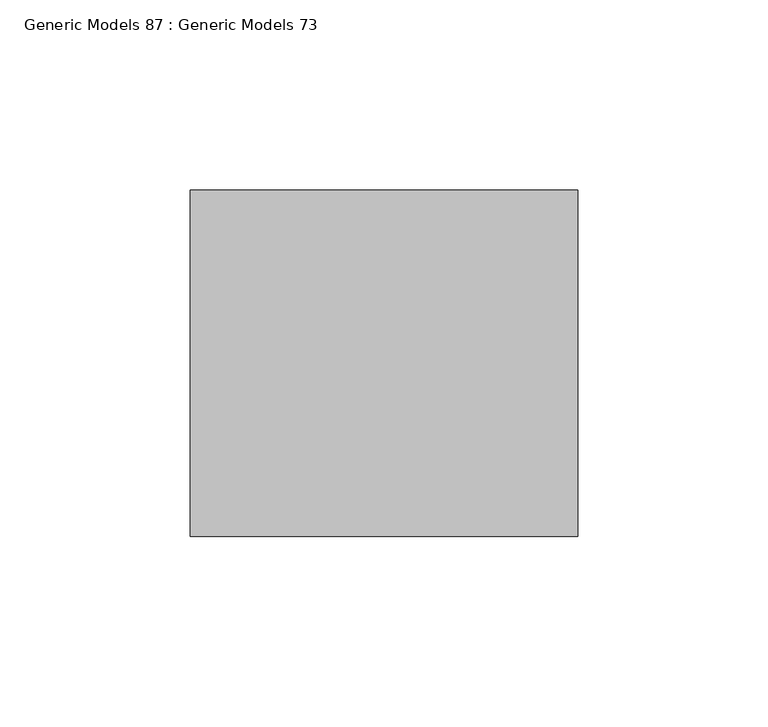
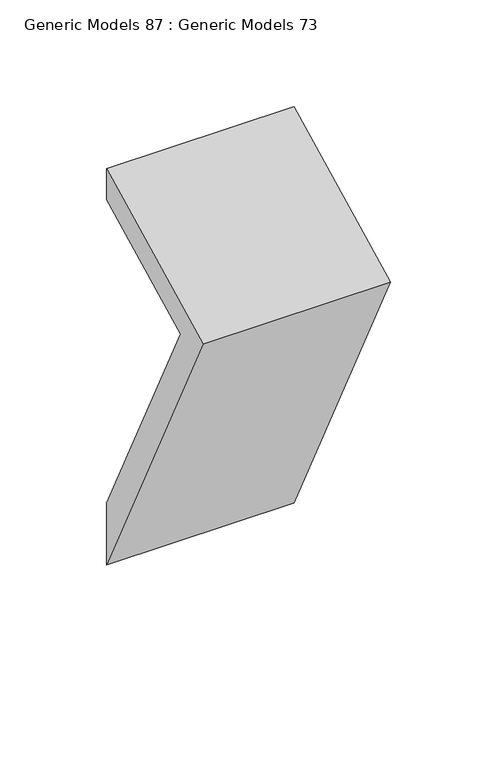
"""IFC4 building model written with IfcOpenShell, lengths in millimetres: proxy geometry, Generic Models 87 : Generic Models 73."""

from ifc_helpers import new_model, si_unit, frame, origin, place, context, project, spatial, polyline, outline, extrude, source, transform, mapped, element, save


def generic_models_87_generic_models_73_a56742e6(model_context):
    return source(origin(), model_context, "Body", "SweptSolid", [
        extrude(outline(polyline([(35114.8094916, 271652.1851052), (35205.6832942, 271697.6220065), (35205.6832942, 271679.8732169), (35136.1080391, 271645.0855894), (35205.6832942, 271505.9350791), (35205.6832942, 271470.4375), (35114.8094916, 271652.1851052)])), frame((31924.6096032, 0.0, 0.0), z_axis=(1.0, 0.0, 0.0), x_axis=(0.0, 1.0, 0.0)), (0.0, 0.0, 1.0), 101.6),
    ])


if __name__ == "__main__":
    model = new_model("IFC4")
    model_context = context("Model", 3, world=origin())
    ifc_project = project(units=[si_unit("LENGTHUNIT", "METRE", prefix="MILLI")], contexts=[model_context])
    site = spatial("IfcSite", under=ifc_project)
    building = spatial("IfcBuilding", under=site)
    placement = place(None, origin())
    generic_models_87_generic_models_73_shape = generic_models_87_generic_models_73_a56742e6(model_context)
    element("IfcBuildingElementProxy", 1, Name="Generic Models 87 : Generic Models 73", ObjectType="Generic Models 87 : Generic Models 73", at=placement, inside=building, context=model_context, shape_type="MappedRepresentation", body=[
        mapped(generic_models_87_generic_models_73_shape, transform((0.0, 0.0, 0.0), x_axis=(1.0, 0.0, 0.0), y_axis=(0.0, 1.0, 0.0), z_axis=(0.0, 0.0, 1.0))),
    ])
    save(model, "model.ifc")

# Revit data of these elements
# Element 1 (IfcBuildingElementProxy, "Generic Models 87 : Generic Models 73")
#   Materials on its faces: "L8 x 4 x 5/8 x 0'-4\" METAL ANGLE"
# Materials
#   "L8 x 4 x 5/8 x 0'-4\" METAL ANGLE": class "Metal", colour RGB 199 199 199, transparency 0, Description = "Carbon steel", Cost = 0
